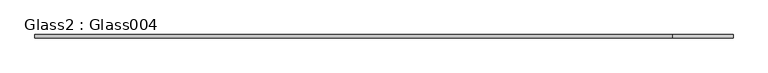
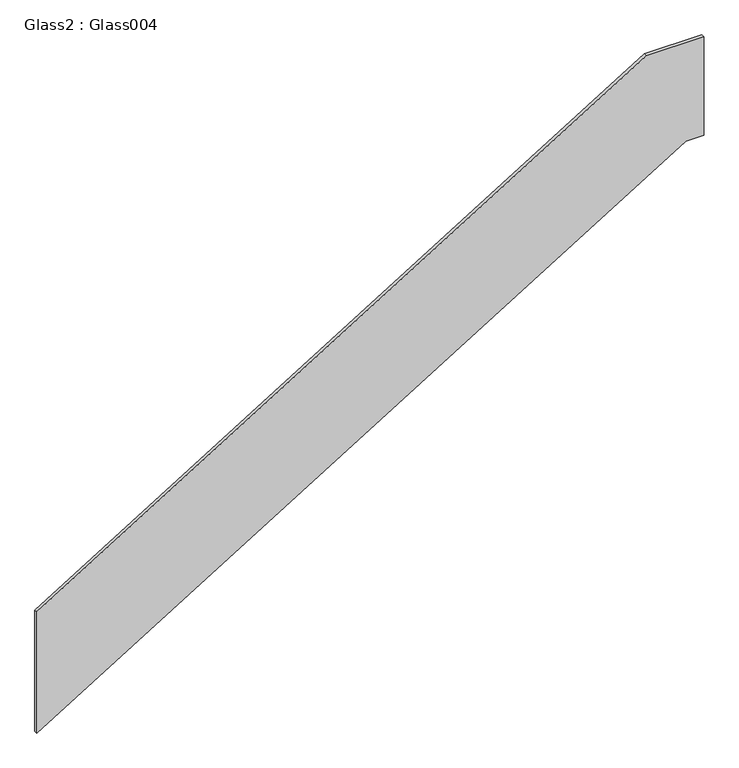
"""IFC4 building model written with IfcOpenShell, lengths in millimetres: proxy geometry, Glass2 : Glass004."""

from ifc_helpers import new_model, si_unit, frame, origin, place, context, project, spatial, polyline, outline, extrude, source, transform, mapped, element, save


def glass2_glass004_a8b2c382(model_context):
    return source(origin(), model_context, "Body", "SweptSolid", [
        extrude(outline(polyline([(38035.9266566, 4990.3637308), (37022.6954344, 4990.3637308), (40173.1410997, 10124.4233335), (40173.1410997, 10267.8101348), (40995.0266566, 10267.8101348), (40995.0266566, 9812.6007679), (38035.9266566, 4990.3637308)])), frame((0.0, 888.7781447, 0.0), z_axis=(0.0, 1.0, 0.0), x_axis=(0.0, 0.0, 1.0)), (0.0, 0.0, 1.0), 25.6840222),
    ])


if __name__ == "__main__":
    model = new_model("IFC4")
    model_context = context("Model", 3, world=origin())
    ifc_project = project(units=[si_unit("LENGTHUNIT", "METRE", prefix="MILLI")], contexts=[model_context])
    site = spatial("IfcSite", under=ifc_project)
    building = spatial("IfcBuilding", under=site)
    placement = place(None, origin())
    glass2_glass004_shape = glass2_glass004_a8b2c382(model_context)
    element("IfcBuildingElementProxy", 1, Name="Glass2 : Glass004", ObjectType="Glass2 : Glass004", at=placement, inside=building, context=model_context, shape_type="MappedRepresentation", body=[
        mapped(glass2_glass004_shape, transform((0.0, 0.0, 0.0), x_axis=(1.0, 0.0, 0.0), y_axis=(0.0, 1.0, 0.0), z_axis=(0.0, 0.0, 1.0))),
    ])
    save(model, "model.ifc")

# Revit data of these elements
# Type "Glass2 : Glass004"
#   NameOverride = "Glass004"
# Element 1 (IfcBuildingElementProxy, "Glass2 : Glass004")
#   Materials on its faces: "1/2\" TEMPERED GLASS"
# Materials
#   "1/2\" TEMPERED GLASS": class "Unassigned", colour RGB 191 240 251, transparency 0, Cost = 0
